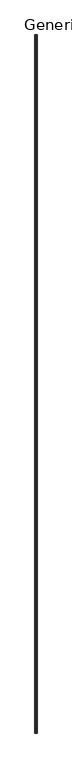
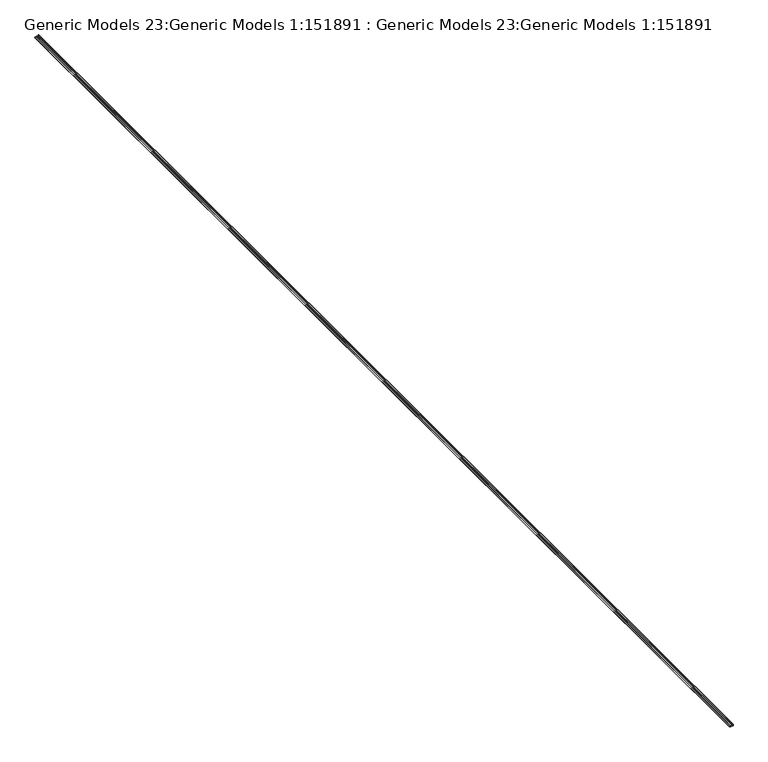
"""IFC4 building model written with IfcOpenShell, lengths in millimetres: proxy geometry, Generic Models 23:Generic Models 1:151891 : Generic Models 23:Generic Models 1:151891."""

from ifc_helpers import new_model, si_unit, frame, origin, place, context, project, spatial, polyline, outline, extrude, source, transform, mapped, element, save


def generic_models_23_generic_models_1_151891_generic_models_23_408cb0b9(model_context):
    return source(origin(), model_context, "Body", "SweptSolid", [
        extrude(outline(polyline([(3048.3048, 8555.233213), (3046.095, 8555.233213), (3046.095, 8535.548213), (3057.525, 8535.548213), (3057.525, 8520.308213), (3046.095, 8520.308213), (3046.095, 8497.8650291), (3044.825, 8497.8650291), (3044.825, 8521.578213), (3056.255, 8521.578213), (3056.255, 8534.278213), (3044.825, 8534.278213), (3044.825, 8556.503213), (3049.5748, 8556.503213), (3049.5748, 8555.6443722), (3068.6193787, 8555.6443722), (3068.6193787, 8554.3743722), (3048.3048, 8554.3743722), (3048.3048, 8555.233213)])), frame((0.0, -6877.9974793, 0.0), z_axis=(0.0, 1.0, 0.0), x_axis=(0.0, 0.0, 1.0)), (0.0, 0.0, 1.0), 19050.0),
    ])


if __name__ == "__main__":
    model = new_model("IFC4")
    model_context = context("Model", 3, world=origin())
    ifc_project = project(units=[si_unit("LENGTHUNIT", "METRE", prefix="MILLI")], contexts=[model_context])
    site = spatial("IfcSite", under=ifc_project)
    building = spatial("IfcBuilding", under=site)
    placement = place(None, origin())
    generic_models_23_generic_models_1_151891_generic_models_23_shape = generic_models_23_generic_models_1_151891_generic_models_23_408cb0b9(model_context)
    element("IfcBuildingElementProxy", 1, Name="Generic Models 23:Generic Models 1:151891 : Generic Models 23:Generic Models 1:151891", ObjectType="Generic Models 23:Generic Models 1:151891 : Generic Models 23:Generic Models 1:151891", at=placement, inside=building, context=model_context, shape_type="MappedRepresentation", body=[
        mapped(generic_models_23_generic_models_1_151891_generic_models_23_shape, transform((0.0, 0.0, 0.0), x_axis=(1.0, 0.0, 0.0), y_axis=(0.0, 1.0, 0.0), z_axis=(0.0, 0.0, 1.0))),
    ])
    save(model, "model.ifc")

# Revit data of these elements
# Type "Generic Models 23:Generic Models 1:151891 : Generic Models 23:Generic Models 1:151891"
#   NameOverride = "Generic Models 23:Generic Models 1:151891"
#   ObjectTypeOverride = "Generic Models 23:Generic Models 1"
#   Reference = "Generic Models 1"
#   Category = "Generic Models"
#   Tag = "151891"
# Element 1 (IfcBuildingElementProxy, "Generic Models 23:Generic Models 1:151891 : Generic Models 23:Generic Models 1:151891")
#   Materials on its faces: "_16 GA. COPPER SOFFIT DRIP SCREED 1359"
# Materials
#   "_16 GA. COPPER SOFFIT DRIP SCREED 1359": class "Unassigned", colour RGB 253 192 103, transparency 0
